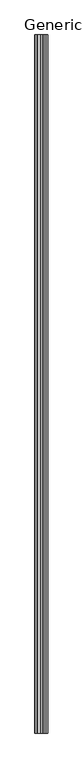
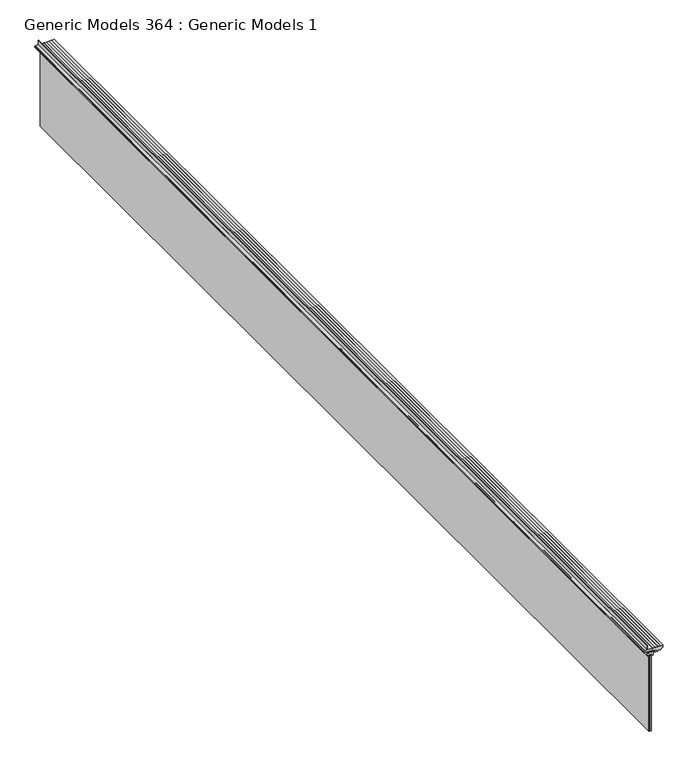
"""IFC4 building model written with IfcOpenShell, lengths in millimetres: proxy geometry, Generic Models 364 : Generic Models 1."""

import ifcopenshell
import ifcopenshell.guid

model = None  # the IFC model being written
_history = None  # IfcOwnerHistory: only IFC2X3 demands one
_inside = {}  # id of a spatial element -> (the spatial element, [elements in it])
_under = {}  # id of a project, library or spatial element -> (it, [spatial elements below it])
_declared = {}  # id of a project -> (the project, [libraries it declares])
_typed = {}  # id of a type object -> (the type object, [elements of that type])
_made_of = {}  # id of a material, layer set ... -> (it, [elements and type objects made of it])


def new_model(schema):
    """Start an empty IFC model of exactly this schema.

    Asked for "IFC4X3", IfcOpenShell would pick the latest addendum, in which some entities
    have other attributes; the version numbers below select the first issue.
    IFC2X3 requires an IfcOwnerHistory on every rooted entity: one is made here for all.
    """
    global model, _history
    if schema == "IFC4X3":
        model = ifcopenshell.file(schema_version=(4, 3, 0, 0))
    else:
        model = ifcopenshell.file(schema=schema)
    _inside.clear()
    _under.clear()
    _declared.clear()
    _typed.clear()
    _made_of.clear()
    _history = None
    if model.schema == "IFC2X3":
        org = make("IfcOrganization", Name="unknown")
        user = make(
            "IfcPersonAndOrganization",
            ThePerson=make("IfcPerson", FamilyName="unknown"),
            TheOrganization=org,
        )
        app = make(
            "IfcApplication",
            ApplicationDeveloper=org,
            Version="unknown",
            ApplicationFullName="unknown",
            ApplicationIdentifier="unknown",
        )
        _history = make(
            "IfcOwnerHistory",
            OwningUser=user,
            OwningApplication=app,
            ChangeAction="ADDED",
            CreationDate=0,
        )
    return model


def make(cls, **values):
    """One entity of the class cls with the attributes given. An attribute that is None is left unset."""
    return model.create_entity(
        cls, **{name: value for name, value in values.items() if value is not None}
    )


def rooted(cls, **values):
    """An entity with a GlobalId (a new one), such as an element, a storey or a relation."""
    return make(cls, GlobalId=ifcopenshell.guid.new(), OwnerHistory=_history, **values)


def si_unit(unit_type, name, prefix=None):
    """IfcSIUnit, for example si_unit("LENGTHUNIT", "METRE", prefix="MILLI")."""
    return make("IfcSIUnit", UnitType=unit_type, Prefix=prefix, Name=name)


def assignment(units):
    """IfcUnitAssignment: the units of a project."""
    return None if units is None else make("IfcUnitAssignment", Units=units)


def point(xyz):
    """IfcCartesianPoint."""
    return None if xyz is None else make("IfcCartesianPoint", Coordinates=xyz)


def direction(xyz):
    """IfcDirection."""
    return None if xyz is None else make("IfcDirection", DirectionRatios=xyz)


def frame(location, z_axis=None, x_axis=None):
    """IfcAxis2Placement3D, a coordinate frame: its origin and axes. An axis left out is left unset."""
    return make(
        "IfcAxis2Placement3D",
        Location=point(location),
        Axis=direction(z_axis),
        RefDirection=direction(x_axis),
    )


def frame_2d(location, x_axis=None):
    """IfcAxis2Placement2D, a coordinate frame in the plane: its origin and x axis."""
    return make(
        "IfcAxis2Placement2D", Location=point(location), RefDirection=direction(x_axis)
    )


def origin():
    """The frame at (0, 0, 0) with its axes left unset."""
    return frame((0.0, 0.0, 0.0))


def place(relative_to, where):
    """IfcLocalPlacement: puts the frame where relative to a parent placement (None: the world)."""
    return make(
        "IfcLocalPlacement", PlacementRelTo=relative_to, RelativePlacement=where
    )


def context(
    kind, dimensions, precision=None, world=None, true_north=None, identifier=None
):
    """IfcGeometricRepresentationContext, for example the 3D "Model" context."""
    return make(
        "IfcGeometricRepresentationContext",
        ContextIdentifier=identifier,
        ContextType=kind,
        CoordinateSpaceDimension=dimensions,
        Precision=precision,
        WorldCoordinateSystem=world,
        TrueNorth=true_north,
    )


def project(units=None, contexts=None):
    """IfcProject with its units and contexts."""
    return rooted(
        "IfcProject",
        Name="project",
        RepresentationContexts=contexts,
        UnitsInContext=assignment(units),
    )


def spatial(cls, under=None, at=None, **own):
    """A site, building, storey or space (cls), placed at a placement, below another one or the project."""
    s = rooted(cls, ObjectPlacement=at, **own)
    if under is not None:
        _under.setdefault(under.id(), (under, []))[1].append(s)
    return s


def polyline(points):
    """IfcPolyline through the points."""
    return make("IfcPolyline", Points=[point(p) for p in points])


def circle_curve(where, radius):
    """IfcCircle in the frame where."""
    return make("IfcCircle", Position=where, Radius=radius)


def trimmed(basis, trim1, trim2, sense, master):
    """IfcTrimmedCurve: the piece of a basis curve between two trims."""
    return make(
        "IfcTrimmedCurve",
        BasisCurve=basis,
        Trim1=trim1,
        Trim2=trim2,
        SenseAgreement=sense,
        MasterRepresentation=master,
    )


def segment(curve, same_sense, transition):
    """IfcCompositeCurveSegment."""
    return make(
        "IfcCompositeCurveSegment",
        Transition=transition,
        SameSense=same_sense,
        ParentCurve=curve,
    )


def composite_curve(segments, self_intersect=None):
    """IfcCompositeCurve: segments joined end to end."""
    return make("IfcCompositeCurve", Segments=segments, SelfIntersect=self_intersect)


def outline(outer, holes=None, kind="AREA"):
    """IfcArbitraryClosedProfileDef: a profile drawn as a closed curve; with holes, ...WithVoids."""
    if holes is None:
        return make("IfcArbitraryClosedProfileDef", ProfileType=kind, OuterCurve=outer)
    return make(
        "IfcArbitraryProfileDefWithVoids",
        ProfileType=kind,
        OuterCurve=outer,
        InnerCurves=holes,
    )


def extrude(swept, where, along, depth):
    """IfcExtrudedAreaSolid: the profile swept, set in the frame where, extruded along a direction by depth."""
    return make(
        "IfcExtrudedAreaSolid",
        SweptArea=swept,
        Position=where,
        ExtrudedDirection=direction(along),
        Depth=depth,
    )


def shape(context_of_items, identifier, shape_type, items):
    """IfcShapeRepresentation: the items that make up one representation, for example the "Body"."""
    return make(
        "IfcShapeRepresentation",
        ContextOfItems=context_of_items,
        RepresentationIdentifier=identifier,
        RepresentationType=shape_type,
        Items=items,
    )


def source(mapping_origin, context_of_items, identifier, shape_type, items):
    """IfcRepresentationMap: a shape defined once, which mapped items show again and again."""
    return make(
        "IfcRepresentationMap",
        MappingOrigin=mapping_origin,
        MappedRepresentation=shape(context_of_items, identifier, shape_type, items),
    )


def transform(
    local_origin,
    x_axis=None,
    y_axis=None,
    z_axis=None,
    scale=None,
    scale2=None,
    scale3=None,
    uniform=True,
):
    """IfcCartesianTransformationOperator3D, or its non-uniform kind. x_axis, y_axis, z_axis: its Axis1, 2, 3."""
    if uniform:
        return make(
            "IfcCartesianTransformationOperator3D",
            Axis1=direction(x_axis),
            Axis2=direction(y_axis),
            LocalOrigin=point(local_origin),
            Scale=scale,
            Axis3=direction(z_axis),
        )
    return make(
        "IfcCartesianTransformationOperator3DnonUniform",
        Axis1=direction(x_axis),
        Axis2=direction(y_axis),
        LocalOrigin=point(local_origin),
        Scale=scale,
        Axis3=direction(z_axis),
        Scale2=scale2,
        Scale3=scale3,
    )


def mapped(mapping_source, mapping_target):
    """IfcMappedItem: shows the shape of a source again, moved by a transform."""
    return make(
        "IfcMappedItem", MappingSource=mapping_source, MappingTarget=mapping_target
    )


def made_of(thing, what):
    """Note that an element or type object is made of a material, layer set ...; save() writes the relation."""
    if what is not None:
        _made_of.setdefault(what.id(), (what, []))[1].append(thing)
    return thing


def element(
    cls,
    number,
    at=None,
    inside=None,
    cuts=None,
    type_object=None,
    material=None,
    context=None,
    identifier="Body",
    shape_type=None,
    held_by="IfcProductDefinitionShape",
    body=None,
    shapes=None,
    **own,
):
    """One element of the class cls, such as IfcWall. Its Tag is "e" and its number.

    at: its placement. inside: the storey or other place that contains it. cuts: it is an
    opening in that element (IfcRelVoidsElement). A single representation is given by context,
    identifier, shape_type and body (its items); several are given by shapes. held_by: the class
    of the entity that holds the representations. save() writes the other relations.
    """
    e = rooted(cls, Tag="e%d" % number, ObjectPlacement=at, **own)
    if body is not None:
        shapes = [shape(context, identifier, shape_type, body)]
    if shapes is not None:
        e.Representation = make(held_by, Representations=shapes)
    if inside is not None:
        _inside.setdefault(inside.id(), (inside, []))[1].append(e)
    if cuts is not None:
        rooted(
            "IfcRelVoidsElement", RelatingBuildingElement=cuts, RelatedOpeningElement=e
        )
    if type_object is not None:
        _typed.setdefault(type_object.id(), (type_object, []))[1].append(e)
    return made_of(e, material)


def aggregate(whole, parts):
    """IfcRelAggregates: a whole, such as a stair, and the parts it consists of."""
    return rooted("IfcRelAggregates", RelatingObject=whole, RelatedObjects=parts)


def save(model, path):
    """Write the relations noted so far, then the file.

    IfcRelAggregates (storeys below a building ...), IfcRelContainedInSpatialStructure (elements
    in a storey), IfcRelDefinesByType, IfcRelAssociatesMaterial and IfcRelDeclares: one each for
    every whole, place, type object, material and project.
    """
    for whole, parts in _under.values():
        aggregate(whole, parts)
    for where, things in _inside.values():
        rooted(
            "IfcRelContainedInSpatialStructure",
            RelatedElements=things,
            RelatingStructure=where,
        )
    for kind, things in _typed.values():
        rooted("IfcRelDefinesByType", RelatedObjects=things, RelatingType=kind)
    for what, things in _made_of.values():
        rooted("IfcRelAssociatesMaterial", RelatedObjects=things, RelatingMaterial=what)
    for by, libraries in _declared.values():
        rooted("IfcRelDeclares", RelatingContext=by, RelatedDefinitions=libraries)
    model.write(path)


def generic_models_364_generic_models_1_7c3e7134(model_context):
    return source(origin(), model_context, "Body", "SweptSolid", [
        extrude(outline(composite_curve([segment(polyline([(129382.901, -83076.4546338), (129382.901, -83094.5231772), (129379.726, -83094.5231772), (129379.726, -83096.8091811), (129382.901, -83096.8091811), (129382.901, -83114.3169303), (129379.726, -83114.3169303), (129379.726, -83116.6029342), (129382.901, -83116.6029342), (129382.901, -83133.6300338), (129380.8182, -83133.6300338), (129380.8182, -83136.8050338), (129382.901, -83136.8050338), (129382.901, -83153.9044164), (129379.726, -83153.9044164), (129379.726, -83156.1904164), (129382.901, -83156.1904164), (129382.901, -83192.6595842), (129418.2728876, -83192.6595842)]), True, "CONTINUOUS"), segment(trimmed(circle_curve(frame_2d((129418.2705467, -83193.3580844)), 0.6985041), [point((129418.2728876, -83192.6595842))], [point((129418.268087, -83194.0565842))], False, "CARTESIAN"), True, "CONTINUOUS"), segment(polyline([(129418.268087, -83194.0565842), (129382.901, -83194.0565842), (129382.901, -83218.9444186), (129381.504, -83218.9444186), (129381.504, -83212.5944186), (129379.218, -83212.5944186), (129379.218, -83220.4979842), (129370.2865767, -83220.4979842), (129367.8642068, -83192.6341842), (129367.8642068, -83157.6837842), (129362.9874142, -83157.6837842), (129362.9874142, -83153.6706571), (129369.4063538, -83153.6706571), (129369.4063538, -83151.6893826), (129361.4561607, -83151.6893826), (129361.4561607, -83143.282047), (129360.5163642, -83143.282047), (129360.5163642, -83125.756047), (129358.2303642, -83125.756047), (129358.2303642, -83143.282047), (129349.5435642, -83143.282047), (129349.5435642, -83146.3300199), (129346.3685642, -83146.3300199), (129346.3685642, -83116.9167958), (129352.7003967, -83116.9167958), (129352.7003967, -83097.8667958), (129355.0879932, -83097.8667958), (129355.0879932, -83096.2666028), (129358.2629932, -83092.3296338), (129358.2629932, -83090.7294408), (129362.2253967, -83090.7294408), (129362.2253967, -83087.5544408), (129363.0381863, -83086.7669888), (129363.0381863, -83076.4546338), (129372.9696053, -83076.4546338), (129372.9696053, -83084.4048268), (129374.9507828, -83084.4048268), (129374.9507828, -83076.4546338), (129382.901, -83076.4546338)]), True, "CONTINUOUS")], self_intersect=False)), frame((0.0, -14323.7036701, 0.0), z_axis=(0.0, 1.0, 0.0), x_axis=(0.0, 0.0, 1.0)), (0.0, 0.0, 1.0), 7886.7),
        extrude(outline(composite_curve([segment(polyline([(129334.0440892, -83184.1577263), (129335.0672312, -83183.1345842), (129338.64785, -83183.1345842), (129338.64785, -83161.6972133), (129336.2595612, -83164.0855022), (129326.3281612, -83164.0855022), (129327.3408112, -83152.2578217), (129329.5031612, -83152.2578217), (129329.5031612, -83148.4899022), (129337.0469612, -83148.4899022), (129337.0469612, -83150.0901022), (129338.64785, -83150.0901022), (129338.64785, -83148.2095842), (129356.93585, -83148.2095842)]), True, "CONTINUOUS"), segment(trimmed(circle_curve(frame_2d((129356.93585, -83149.0223842)), 0.8128), [point((129356.93585, -83148.2095842))], [point((129357.74865, -83149.0223842))], False, "CARTESIAN"), True, "CONTINUOUS"), segment(polyline([(129357.74865, -83149.0223842), (129357.74865, -83162.3573842)]), True, "CONTINUOUS"), segment(trimmed(circle_curve(frame_2d((129357.74865, -83164.3385842)), 1.9812), [point((129357.74865, -83162.3573842))], [point((129357.74865, -83166.3197842))], True, "CARTESIAN"), True, "CONTINUOUS"), segment(polyline([(129357.74865, -83166.3197842), (129357.74865, -83178.5117842), (129363.05725, -83178.5117842), (129363.05725, -83184.1251842), (129355.13245, -83184.1251842), (129355.13245, -83186.0301842), (129358.43445, -83186.0301842), (129358.43445, -83187.7065842), (129360.46645, -83187.7065842), (129360.46645, -83190.2719842)]), True, "CONTINUOUS"), segment(trimmed(circle_curve(frame_2d((129358.07885, -83190.2719842)), 2.3876), [point((129360.46645, -83190.2719842))], [point((129358.07885, -83192.6595842))], False, "CARTESIAN"), True, "CONTINUOUS"), segment(polyline([(129358.07885, -83192.6595842), (129335.77765, -83192.6595842), (129335.77765, -83190.2719842), (129327.9718265, -83187.7366236), (129327.7822762, -83185.2935842), (129329.80865, -83185.2935842), (129329.80865, -83184.1577263), (129334.0440892, -83184.1577263)]), True, "CONTINUOUS")], self_intersect=False)), frame((0.0, -14323.7036701, 0.0), z_axis=(0.0, 1.0, 0.0), x_axis=(0.0, 0.0, 1.0)), (0.0, 0.0, 1.0), 7886.7),
        extrude(outline(polyline([(-83164.8792522, -14323.7036701), (-83169.6417522, -14323.7036701), (-83169.6417522, -6437.0036701), (-83164.8792522, -6437.0036701), (-83164.8792522, -14323.7036701)])), frame((0.0, 0.0, 128735.516552), z_axis=(0.0, 0.0, 1.0), x_axis=(1.0, 0.0, 0.0)), (0.0, 0.0, 1.0), 602.3375481),
        extrude(outline(polyline([(-83170.4355022, -14323.7036701), (-83176.7845842, -14323.7036701), (-83176.7845842, -6437.0036701), (-83170.4355022, -6437.0036701), (-83170.4355022, -14323.7036701)])), frame((0.0, 0.0, 129331.5041), z_axis=(0.0, 0.0, 1.0), x_axis=(1.0, 0.0, 0.0)), (0.0, 0.0, 1.0), 6.35),
        extrude(outline(polyline([(-83177.5783342, -14323.7036701), (-83182.3408342, -14323.7036701), (-83182.3408342, -6437.0036701), (-83177.5783342, -6437.0036701), (-83177.5783342, -14323.7036701)])), frame((0.0, 0.0, 128735.516552), z_axis=(0.0, 0.0, 1.0), x_axis=(1.0, 0.0, 0.0)), (0.0, 0.0, 1.0), 602.3375481),
    ])


if __name__ == "__main__":
    model = new_model("IFC4")
    model_context = context("Model", 3, world=origin())
    ifc_project = project(units=[si_unit("LENGTHUNIT", "METRE", prefix="MILLI")], contexts=[model_context])
    site = spatial("IfcSite", under=ifc_project)
    building = spatial("IfcBuilding", under=site)
    placement = place(None, origin())
    generic_models_364_generic_models_1_shape = generic_models_364_generic_models_1_7c3e7134(model_context)
    element("IfcBuildingElementProxy", 1, Name="Generic Models 364 : Generic Models 1", ObjectType="Generic Models 364 : Generic Models 1", at=placement, inside=building, context=model_context, shape_type="MappedRepresentation", body=[
        mapped(generic_models_364_generic_models_1_shape, transform((0.0, 0.0, 0.0), x_axis=(1.0, 0.0, 0.0), y_axis=(0.0, 1.0, 0.0), z_axis=(0.0, 0.0, 1.0))),
    ])
    save(model, "model.ifc")

# Revit data of these elements
# Element 1 (IfcBuildingElementProxy, "Generic Models 364 : Generic Models 1")
#   Materials on its faces: "_WINDOW PER SCHEDULE"
# Materials
#   "_WINDOW PER SCHEDULE": class "Generic", colour RGB 255 255 255, transparency 0, Cost = 0
